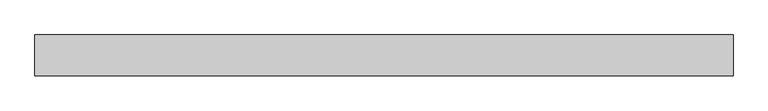
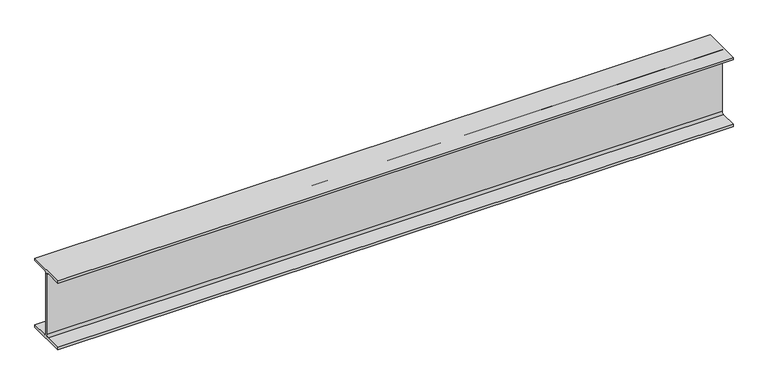
"""IFC4 building model written with IfcOpenShell, lengths in millimetres: beam geometry, Old_Steel Beam_H-KSD3502 : H_SB_ASB_H-250×125x6x9."""

from ifc_helpers import new_model, si_unit, point, frame, frame_2d, origin, place, context, project, spatial, polyline, circle_curve, trimmed, segment, composite_curve, outline, extrude, source, transform, mapped, element, save


def beam_219eb426(model_context):
    return source(origin(), model_context, "Body", "SweptSolid", [
        extrude(outline(composite_curve([segment(polyline([(82.5, -141.5), (82.5, -151.7), (-82.5, -151.7), (-82.5, -141.5), (-11.9, -141.5)]), True, "CONTINUOUS"), segment(trimmed(circle_curve(frame_2d((-11.9, -132.6)), 8.9), [point((-11.9, -141.5))], [point((-3.0, -132.6))], True, "CARTESIAN"), True, "CONTINUOUS"), segment(polyline([(-3.0, -132.6), (-3.0, 132.6)]), True, "CONTINUOUS"), segment(trimmed(circle_curve(frame_2d((-11.9, 132.6)), 8.9), [point((-3.0, 132.6))], [point((-11.9, 141.5))], True, "CARTESIAN"), True, "CONTINUOUS"), segment(polyline([(-11.9, 141.5), (-82.5, 141.5), (-82.5, 151.7), (82.5, 151.7), (82.5, 141.5), (11.9, 141.5)]), True, "CONTINUOUS"), segment(trimmed(circle_curve(frame_2d((11.9, 132.6)), 8.9), [point((11.9, 141.5))], [point((3.0, 132.6))], True, "CARTESIAN"), True, "CONTINUOUS"), segment(polyline([(3.0, 132.6), (3.0, -132.6)]), True, "CONTINUOUS"), segment(trimmed(circle_curve(frame_2d((11.9, -132.6)), 8.9), [point((3.0, -132.6))], [point((11.9, -141.5))], True, "CARTESIAN"), True, "CONTINUOUS"), segment(polyline([(11.9, -141.5), (82.5, -141.5)]), True, "CONTINUOUS")], self_intersect=False)), frame((-1404.8, 0.0, 0.0), z_axis=(1.0, 0.0, 0.0), x_axis=(0.0, 1.0, 0.0)), (0.0, 0.0, 1.0), 2809.6),
    ])


if __name__ == "__main__":
    model = new_model("IFC4")
    model_context = context("Model", 3, world=origin())
    ifc_project = project(units=[si_unit("LENGTHUNIT", "METRE", prefix="MILLI")], contexts=[model_context])
    site = spatial("IfcSite", under=ifc_project)
    building = spatial("IfcBuilding", under=site)
    placement = place(None, origin())
    beam_shape = beam_219eb426(model_context)
    element("IfcBeam", 1, ObjectType="Old_Steel Beam_H-KSD3502 : H_SB_ASB_H-250×125x6x9", at=placement, inside=building, context=model_context, shape_type="MappedRepresentation", body=[
        mapped(beam_shape, transform((0.0, 0.0, 0.0), x_axis=(1.0, 0.0, 0.0), y_axis=(0.0, 1.0, 0.0), z_axis=(0.0, 0.0, 1.0))),
    ])
    save(model, "model.ifc")

# Revit data of these elements
# Type "Old_Steel Beam_H-KSD3502 : H_SB_ASB_H-250×125x6x9"
#   Width = 12.5 cm
#   Web Thickness = 0.6 cm
#   Web Fillet = 1.2 cm
#   Warping Constant = 42539.8 cm⁶
#   Torsional Moment of Inertia = 7.8102 cm⁴
#   Torsional Modulus = 1.0 cm³
#   Section Area = 37.66 cm²
#   Plastic Modulus weak axis = 73.1 cm³
#   Plastic Modulus strong axis = 366.0 cm³
#   Perimeter = 0.97 m²/m
#   Nominal Weight = 29.60 kgf/m
#   Moment of Inertia weak axis = 294.00 cm⁴
#   Moment of Inertia strong axis = 4050.00 cm⁴
#   Height = 25.0 cm
#   Flange Thickness = 0.9 cm
#   Elastic Modulus weak axis = 47.0 cm³
#   Elastic Modulus strong axis = 324.0 cm³
#   Centroid Vertical = 12.5 cm
#   Centroid Horizontal = 6.25 cm
#   Length [instance default] = 1.5240 m
#   Structural Material [instance default] = Steel, 45-345
#   Assembly Code = ""
# Element 1 (IfcBeam, "Old_Steel Beam_H-KSD3502 : H_SB_ASB_H-250×125x6x9")
#   Structural Material = none
# Materials
#   "Steel, 45-345": class "Metal", colour RGB 189 187 185, transparency 0, Description = "Steel 345 MPa", Cost = 0
